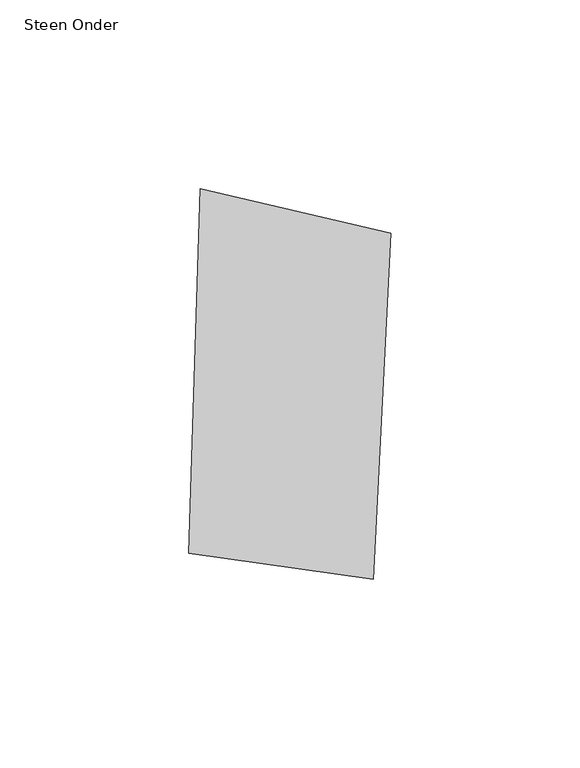
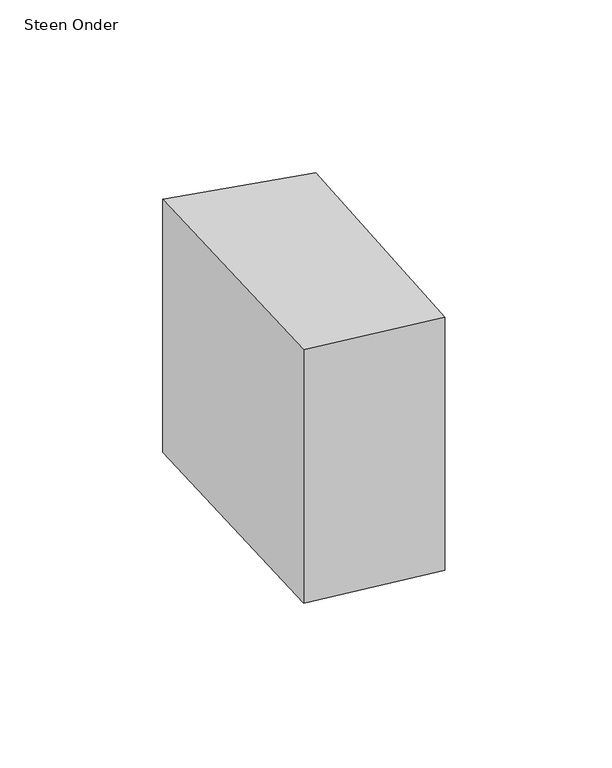
"""IFC4 building model written with IfcOpenShell, lengths in millimetres: proxy geometry, 00_GMA_steen_versie_4 : Steen Onder."""

from ifc_helpers import new_model, si_unit, origin, origin_with_axes, place, context, project, spatial, polyline, outline, extrude, source, transform, mapped, element, save


def steen_onder_d39f949e(model_context):
    return source(origin(), model_context, "Body", "SweptSolid", [
        extrude(outline(polyline([(102.8506172, 112.8815379), (98.2227221, 21.4004251), (49.3993657, 28.1957753), (52.4323172, 124.6763915), (102.8506172, 112.8815379)])), origin_with_axes(), (0.0, 0.0, 1.0), 100.0),
    ])


if __name__ == "__main__":
    model = new_model("IFC4")
    model_context = context("Model", 3, world=origin())
    ifc_project = project(units=[si_unit("LENGTHUNIT", "METRE", prefix="MILLI")], contexts=[model_context])
    site = spatial("IfcSite", under=ifc_project)
    building = spatial("IfcBuilding", under=site)
    placement = place(None, origin())
    steen_onder_shape = steen_onder_d39f949e(model_context)
    element("IfcBuildingElementProxy", 1, Name="00_GMA_steen_versie_4 : Steen Onder", ObjectType="00_GMA_steen_versie_4 : Steen Onder", at=placement, inside=building, context=model_context, shape_type="MappedRepresentation", body=[
        mapped(steen_onder_shape, transform((0.0, 0.0, 0.0), x_axis=(1.0, 0.0, 0.0), y_axis=(0.0, 1.0, 0.0), z_axis=(0.0, 0.0, 1.0))),
    ])
    save(model, "model.ifc")

# Revit data of these elements
# Type "00_GMA_steen_versie_4 : Steen Onder"
#   StootVoegHalfBoven [instance default] = 5 mm
#   StootVoegHalf [instance default] = 5 mm
#   StootVoegBreedteOnder = 10 mm
#   StootVoegBreedteBoven = 10 mm
#   Steendikte = 100 mm
#   LintVoegOnderHalf = 0 mm
#   LintVoegOnder = 0 mm
#   LintVoegBovenHalf = 5 mm
#   LintVoegBoven = 10 mm
#   materiaal = none
#   MateriaalVoeg = none
#   Default Elevation = 0
